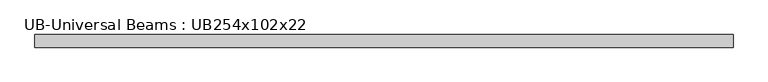
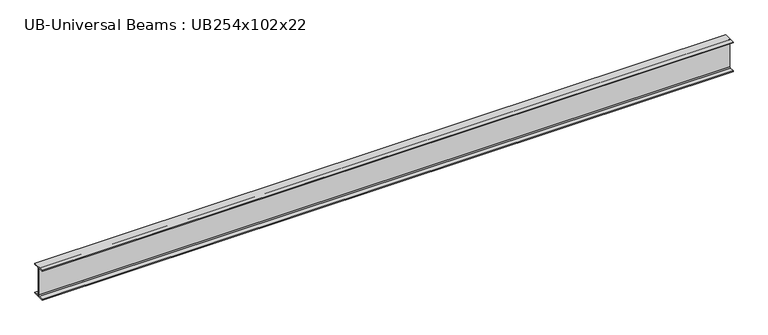
"""IFC4 building model written with IfcOpenShell, lengths in millimetres: beam geometry, UB-Universal Beams : UB254x102x22."""

from ifc_helpers import new_model, si_unit, point, frame, frame_2d, origin, place, context, project, spatial, polyline, circle_curve, trimmed, segment, composite_curve, outline, extrude, source, transform, mapped, element, save


def ub_universal_beams_ub254x102x22_6668b1ee(model_context):
    return source(origin(), model_context, "Body", "SweptSolid", [
        extrude(outline(composite_curve([segment(polyline([(50.8, -120.2), (50.8, -127.0), (-50.8, -127.0), (-50.8, -120.2), (-10.45, -120.2)]), True, "CONTINUOUS"), segment(trimmed(circle_curve(frame_2d((-10.45, -112.6)), 7.6), [point((-10.45, -120.2))], [point((-2.85, -112.6))], True, "CARTESIAN"), True, "CONTINUOUS"), segment(polyline([(-2.85, -112.6), (-2.85, 112.6)]), True, "CONTINUOUS"), segment(trimmed(circle_curve(frame_2d((-10.45, 112.6)), 7.6), [point((-2.85, 112.6))], [point((-10.45, 120.2))], True, "CARTESIAN"), True, "CONTINUOUS"), segment(polyline([(-10.45, 120.2), (-50.8, 120.2), (-50.8, 127.0), (50.8, 127.0), (50.8, 120.2), (10.45, 120.2)]), True, "CONTINUOUS"), segment(trimmed(circle_curve(frame_2d((10.45, 112.6)), 7.6), [point((10.45, 120.2))], [point((2.85, 112.6))], True, "CARTESIAN"), True, "CONTINUOUS"), segment(polyline([(2.85, 112.6), (2.85, -112.6)]), True, "CONTINUOUS"), segment(trimmed(circle_curve(frame_2d((10.45, -112.6)), 7.6), [point((2.85, -112.6))], [point((10.45, -120.2))], True, "CARTESIAN"), True, "CONTINUOUS"), segment(polyline([(10.45, -120.2), (50.8, -120.2)]), True, "CONTINUOUS")], self_intersect=False)), frame((-2762.4, 0.0, 0.0), z_axis=(1.0, 0.0, 0.0), x_axis=(0.0, 1.0, 0.0)), (0.0, 0.0, 1.0), 5597.1),
    ])


if __name__ == "__main__":
    model = new_model("IFC4")
    model_context = context("Model", 3, world=origin())
    ifc_project = project(units=[si_unit("LENGTHUNIT", "METRE", prefix="MILLI")], contexts=[model_context])
    site = spatial("IfcSite", under=ifc_project)
    building = spatial("IfcBuilding", under=site)
    placement = place(None, origin())
    ub_universal_beams_ub254x102x22_shape = ub_universal_beams_ub254x102x22_6668b1ee(model_context)
    element("IfcBeam", 1, ObjectType="UB-Universal Beams : UB254x102x22", at=placement, inside=building, context=model_context, shape_type="MappedRepresentation", body=[
        mapped(ub_universal_beams_ub254x102x22_shape, transform((0.0, 0.0, 0.0), x_axis=(1.0, 0.0, 0.0), y_axis=(0.0, 1.0, 0.0), z_axis=(0.0, 0.0, 1.0))),
    ])
    save(model, "model.ifc")

# Revit data of these elements
# Type "UB-Universal Beams : UB254x102x22"
#   Section Name Key = "UB254X102X22"
#   Width = 10.16 cm
#   Web Thickness = 0.57 cm
#   Web Fillet = 0.76 cm
#   Warping Constant = 18200.0 cm⁶
#   Torsional Moment of Inertia = 4.15 cm⁴
#   Section Area = 28.0 cm²
#   Plastic Modulus weak axis = 37.3 cm³
#   Plastic Modulus strong axis = 259.0 cm³
#   Nominal Weight = 22.00 kgf/m
#   Moment of Inertia weak axis = 119.00 cm⁴
#   Moment of Inertia strong axis = 2841.00 cm⁴
#   Height = 25.4 cm
#   Flange Thickness = 0.68 cm
#   Elastic Modulus weak axis = 23.5 cm³
#   Elastic Modulus strong axis = 224.0 cm³
#   Centroid Vertical = 12.7 cm
#   Centroid Horizontal = 5.08 cm
#   Bolt Spacing = 5.4 cm
#   Length [instance default] = 1500 mm
#   Structural Material [instance default] = Metal - Steel 43-275
#   Type Comments = ""
#   Assembly Code = ""
# Element 1 (IfcBeam, "UB-Universal Beams : UB254x102x22")
#   Materials on its faces: "Metal - Steel 43-275"
# Materials
#   "Metal - Steel 43-275": class "Metal", colour RGB 247 247 247, transparency 0, Cost = 0
